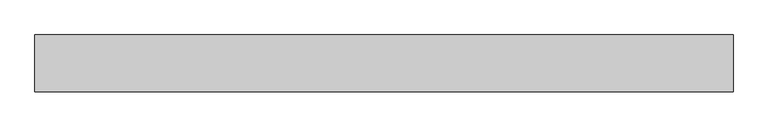
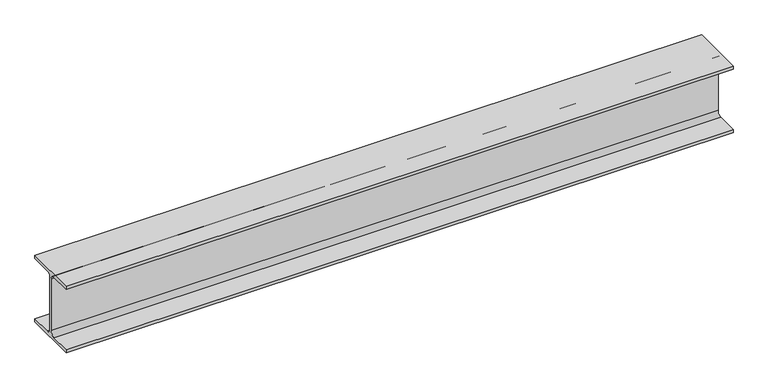
"""IFC4 building model written with IfcOpenShell, lengths in millimetres: beam geometry, 0912_Steel Framing_H-KSD3502 : H_SB_ASB_H-194x150x6x9."""

from ifc_helpers import new_model, si_unit, point, frame, frame_2d, origin, place, context, project, spatial, polyline, circle_curve, trimmed, segment, composite_curve, outline, extrude, source, transform, mapped, element, save


def beam_6f81609b(model_context):
    return source(origin(), model_context, "Body", "SweptSolid", [
        extrude(outline(composite_curve([segment(polyline([(75.0, -88.0), (75.0, -97.0), (-75.0, -97.0), (-75.0, -88.0), (-16.0, -88.0)]), True, "CONTINUOUS"), segment(trimmed(circle_curve(frame_2d((-16.0, -75.0)), 13.0), [point((-16.0, -88.0))], [point((-3.0, -75.0))], True, "CARTESIAN"), True, "CONTINUOUS"), segment(polyline([(-3.0, -75.0), (-3.0, 75.0)]), True, "CONTINUOUS"), segment(trimmed(circle_curve(frame_2d((-16.0, 75.0)), 13.0), [point((-3.0, 75.0))], [point((-16.0, 88.0))], True, "CARTESIAN"), True, "CONTINUOUS"), segment(polyline([(-16.0, 88.0), (-75.0, 88.0), (-75.0, 97.0), (75.0, 97.0), (75.0, 88.0), (16.0, 88.0)]), True, "CONTINUOUS"), segment(trimmed(circle_curve(frame_2d((16.0, 75.0)), 13.0), [point((16.0, 88.0))], [point((3.0, 75.0))], True, "CARTESIAN"), True, "CONTINUOUS"), segment(polyline([(3.0, 75.0), (3.0, -75.0)]), True, "CONTINUOUS"), segment(trimmed(circle_curve(frame_2d((16.0, -75.0)), 13.0), [point((3.0, -75.0))], [point((16.0, -88.0))], True, "CARTESIAN"), True, "CONTINUOUS"), segment(polyline([(16.0, -88.0), (75.0, -88.0)]), True, "CONTINUOUS")], self_intersect=False)), frame((-851.3274068, 0.0, 0.0), z_axis=(1.0, 0.0, 0.0), x_axis=(0.0, 1.0, 0.0)), (0.0, 0.0, 1.0), 1839.6820153),
    ])


if __name__ == "__main__":
    model = new_model("IFC4")
    model_context = context("Model", 3, world=origin())
    ifc_project = project(units=[si_unit("LENGTHUNIT", "METRE", prefix="MILLI")], contexts=[model_context])
    site = spatial("IfcSite", under=ifc_project)
    building = spatial("IfcBuilding", under=site)
    placement = place(None, origin())
    beam_shape = beam_6f81609b(model_context)
    element("IfcBeam", 1, ObjectType="0912_Steel Framing_H-KSD3502 : H_SB_ASB_H-194x150x6x9", at=placement, inside=building, context=model_context, shape_type="MappedRepresentation", body=[
        mapped(beam_shape, transform((0.0, 0.0, 0.0), x_axis=(1.0, 0.0, 0.0), y_axis=(0.0, 1.0, 0.0), z_axis=(0.0, 0.0, 1.0))),
    ])
    save(model, "model.ifc")

# Revit data of these elements
# Type "0912_Steel Framing_H-KSD3502 : H_SB_ASB_H-194x150x6x9"
#   H_WM Code_1 = "S01AA002-00001 | Main Steel Structure Fabrication Work | Shelter/Building | Medium Steel - Standard (90KG/M>Weight≥30KG/M) | Material: (   )"
#   H_WM Code_2 = "S03AA028-00001 | Main Steel Structure Erection Work | Shelter/Building | Medium Steel (90KG/M>Weight≥30KG/M) | Material: (   )"
#   H_WM Code_3 = "S01AA010-00001 | Main Steel Structure Fabrication Work | Shelter/Building | Steel Painting/Coating | for Non-Fireproofed Steel Surface, Surface Preparation, Primer, Second & Final Coat | Material: (   )"
#   H_Q'ty Cal Type Tag = "SB-Q2"
#   Width = 15.0 cm
#   Web Thickness = 0.6 cm
#   Web Fillet = 1.3 cm
#   Warping Constant = 43316.0 cm⁶
#   W = 0
#   Torsional Moment of Inertia = 8.622 cm⁴
#   Section Area = 39.01 cm²
#   Plastic Modulus weak axis = 104.0 cm³
#   Plastic Modulus strong axis = 309.0 cm³
#   Perimeter = 0.95 m²/m
#   Nominal Weight = 30.60 kgf/m
#   Moment of Inertia weak axis = 507.00 cm⁴
#   Moment of Inertia strong axis = 2690.00 cm⁴
#   Height = 19.4 cm
#   Flange Thickness = 0.9 cm
#   Elastic Modulus weak axis = 67.6 cm³
#   Elastic Modulus strong axis = 277.0 cm³
#   Centroid Vertical = 9.7 cm
#   Centroid Horizontal = 7.5 cm
#   Ix = 26900000
#   Length [instance default] = 1.5240 m
#   Zx = 309000
#   b = 0.1500 m
#   h = 0.1940 m
#   r = 0.0130 m
#   s = 0.0060 m
#   t = 0.0090 m
#   A = 0.003901 m²
#   Structural Material [instance default] = Steel, 45-345
#   Assembly Code = ""
# Element 1 (IfcBeam, "0912_Steel Framing_H-KSD3502 : H_SB_ASB_H-194x150x6x9")
#   Structural Material = none
# Materials
#   "Steel, 45-345": class "Metal", colour RGB 189 187 185, transparency 0, Description = "Steel 345 MPa", Cost = 0
